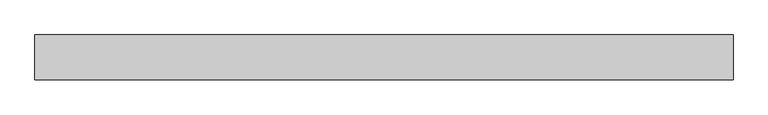
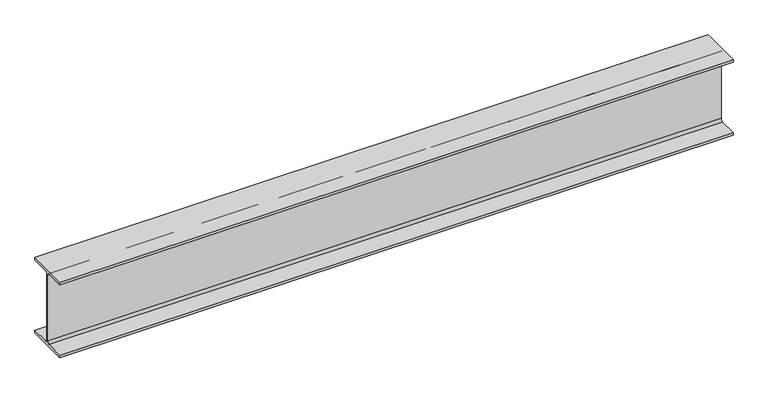
"""IFC4 building model written with IfcOpenShell, lengths in millimetres: beam geometry, Old_Steel Beam_H-KSD3502 : H_SB_ASB_H-350×175x7x11."""

import ifcopenshell
import ifcopenshell.guid

model = None  # the IFC model being written
_history = None  # IfcOwnerHistory: only IFC2X3 demands one
_inside = {}  # id of a spatial element -> (the spatial element, [elements in it])
_under = {}  # id of a project, library or spatial element -> (it, [spatial elements below it])
_declared = {}  # id of a project -> (the project, [libraries it declares])
_typed = {}  # id of a type object -> (the type object, [elements of that type])
_made_of = {}  # id of a material, layer set ... -> (it, [elements and type objects made of it])


def new_model(schema):
    """Start an empty IFC model of exactly this schema.

    Asked for "IFC4X3", IfcOpenShell would pick the latest addendum, in which some entities
    have other attributes; the version numbers below select the first issue.
    IFC2X3 requires an IfcOwnerHistory on every rooted entity: one is made here for all.
    """
    global model, _history
    if schema == "IFC4X3":
        model = ifcopenshell.file(schema_version=(4, 3, 0, 0))
    else:
        model = ifcopenshell.file(schema=schema)
    _inside.clear()
    _under.clear()
    _declared.clear()
    _typed.clear()
    _made_of.clear()
    _history = None
    if model.schema == "IFC2X3":
        org = make("IfcOrganization", Name="unknown")
        user = make(
            "IfcPersonAndOrganization",
            ThePerson=make("IfcPerson", FamilyName="unknown"),
            TheOrganization=org,
        )
        app = make(
            "IfcApplication",
            ApplicationDeveloper=org,
            Version="unknown",
            ApplicationFullName="unknown",
            ApplicationIdentifier="unknown",
        )
        _history = make(
            "IfcOwnerHistory",
            OwningUser=user,
            OwningApplication=app,
            ChangeAction="ADDED",
            CreationDate=0,
        )
    return model


def make(cls, **values):
    """One entity of the class cls with the attributes given. An attribute that is None is left unset."""
    return model.create_entity(
        cls, **{name: value for name, value in values.items() if value is not None}
    )


def rooted(cls, **values):
    """An entity with a GlobalId (a new one), such as an element, a storey or a relation."""
    return make(cls, GlobalId=ifcopenshell.guid.new(), OwnerHistory=_history, **values)


def si_unit(unit_type, name, prefix=None):
    """IfcSIUnit, for example si_unit("LENGTHUNIT", "METRE", prefix="MILLI")."""
    return make("IfcSIUnit", UnitType=unit_type, Prefix=prefix, Name=name)


def assignment(units):
    """IfcUnitAssignment: the units of a project."""
    return None if units is None else make("IfcUnitAssignment", Units=units)


def point(xyz):
    """IfcCartesianPoint."""
    return None if xyz is None else make("IfcCartesianPoint", Coordinates=xyz)


def direction(xyz):
    """IfcDirection."""
    return None if xyz is None else make("IfcDirection", DirectionRatios=xyz)


def frame(location, z_axis=None, x_axis=None):
    """IfcAxis2Placement3D, a coordinate frame: its origin and axes. An axis left out is left unset."""
    return make(
        "IfcAxis2Placement3D",
        Location=point(location),
        Axis=direction(z_axis),
        RefDirection=direction(x_axis),
    )


def frame_2d(location, x_axis=None):
    """IfcAxis2Placement2D, a coordinate frame in the plane: its origin and x axis."""
    return make(
        "IfcAxis2Placement2D", Location=point(location), RefDirection=direction(x_axis)
    )


def origin():
    """The frame at (0, 0, 0) with its axes left unset."""
    return frame((0.0, 0.0, 0.0))


def place(relative_to, where):
    """IfcLocalPlacement: puts the frame where relative to a parent placement (None: the world)."""
    return make(
        "IfcLocalPlacement", PlacementRelTo=relative_to, RelativePlacement=where
    )


def context(
    kind, dimensions, precision=None, world=None, true_north=None, identifier=None
):
    """IfcGeometricRepresentationContext, for example the 3D "Model" context."""
    return make(
        "IfcGeometricRepresentationContext",
        ContextIdentifier=identifier,
        ContextType=kind,
        CoordinateSpaceDimension=dimensions,
        Precision=precision,
        WorldCoordinateSystem=world,
        TrueNorth=true_north,
    )


def project(units=None, contexts=None):
    """IfcProject with its units and contexts."""
    return rooted(
        "IfcProject",
        Name="project",
        RepresentationContexts=contexts,
        UnitsInContext=assignment(units),
    )


def spatial(cls, under=None, at=None, **own):
    """A site, building, storey or space (cls), placed at a placement, below another one or the project."""
    s = rooted(cls, ObjectPlacement=at, **own)
    if under is not None:
        _under.setdefault(under.id(), (under, []))[1].append(s)
    return s


def polyline(points):
    """IfcPolyline through the points."""
    return make("IfcPolyline", Points=[point(p) for p in points])


def circle_curve(where, radius):
    """IfcCircle in the frame where."""
    return make("IfcCircle", Position=where, Radius=radius)


def trimmed(basis, trim1, trim2, sense, master):
    """IfcTrimmedCurve: the piece of a basis curve between two trims."""
    return make(
        "IfcTrimmedCurve",
        BasisCurve=basis,
        Trim1=trim1,
        Trim2=trim2,
        SenseAgreement=sense,
        MasterRepresentation=master,
    )


def segment(curve, same_sense, transition):
    """IfcCompositeCurveSegment."""
    return make(
        "IfcCompositeCurveSegment",
        Transition=transition,
        SameSense=same_sense,
        ParentCurve=curve,
    )


def composite_curve(segments, self_intersect=None):
    """IfcCompositeCurve: segments joined end to end."""
    return make("IfcCompositeCurve", Segments=segments, SelfIntersect=self_intersect)


def outline(outer, holes=None, kind="AREA"):
    """IfcArbitraryClosedProfileDef: a profile drawn as a closed curve; with holes, ...WithVoids."""
    if holes is None:
        return make("IfcArbitraryClosedProfileDef", ProfileType=kind, OuterCurve=outer)
    return make(
        "IfcArbitraryProfileDefWithVoids",
        ProfileType=kind,
        OuterCurve=outer,
        InnerCurves=holes,
    )


def extrude(swept, where, along, depth):
    """IfcExtrudedAreaSolid: the profile swept, set in the frame where, extruded along a direction by depth."""
    return make(
        "IfcExtrudedAreaSolid",
        SweptArea=swept,
        Position=where,
        ExtrudedDirection=direction(along),
        Depth=depth,
    )


def shape(context_of_items, identifier, shape_type, items):
    """IfcShapeRepresentation: the items that make up one representation, for example the "Body"."""
    return make(
        "IfcShapeRepresentation",
        ContextOfItems=context_of_items,
        RepresentationIdentifier=identifier,
        RepresentationType=shape_type,
        Items=items,
    )


def source(mapping_origin, context_of_items, identifier, shape_type, items):
    """IfcRepresentationMap: a shape defined once, which mapped items show again and again."""
    return make(
        "IfcRepresentationMap",
        MappingOrigin=mapping_origin,
        MappedRepresentation=shape(context_of_items, identifier, shape_type, items),
    )


def transform(
    local_origin,
    x_axis=None,
    y_axis=None,
    z_axis=None,
    scale=None,
    scale2=None,
    scale3=None,
    uniform=True,
):
    """IfcCartesianTransformationOperator3D, or its non-uniform kind. x_axis, y_axis, z_axis: its Axis1, 2, 3."""
    if uniform:
        return make(
            "IfcCartesianTransformationOperator3D",
            Axis1=direction(x_axis),
            Axis2=direction(y_axis),
            LocalOrigin=point(local_origin),
            Scale=scale,
            Axis3=direction(z_axis),
        )
    return make(
        "IfcCartesianTransformationOperator3DnonUniform",
        Axis1=direction(x_axis),
        Axis2=direction(y_axis),
        LocalOrigin=point(local_origin),
        Scale=scale,
        Axis3=direction(z_axis),
        Scale2=scale2,
        Scale3=scale3,
    )


def mapped(mapping_source, mapping_target):
    """IfcMappedItem: shows the shape of a source again, moved by a transform."""
    return make(
        "IfcMappedItem", MappingSource=mapping_source, MappingTarget=mapping_target
    )


def made_of(thing, what):
    """Note that an element or type object is made of a material, layer set ...; save() writes the relation."""
    if what is not None:
        _made_of.setdefault(what.id(), (what, []))[1].append(thing)
    return thing


def element(
    cls,
    number,
    at=None,
    inside=None,
    cuts=None,
    type_object=None,
    material=None,
    context=None,
    identifier="Body",
    shape_type=None,
    held_by="IfcProductDefinitionShape",
    body=None,
    shapes=None,
    **own,
):
    """One element of the class cls, such as IfcWall. Its Tag is "e" and its number.

    at: its placement. inside: the storey or other place that contains it. cuts: it is an
    opening in that element (IfcRelVoidsElement). A single representation is given by context,
    identifier, shape_type and body (its items); several are given by shapes. held_by: the class
    of the entity that holds the representations. save() writes the other relations.
    """
    e = rooted(cls, Tag="e%d" % number, ObjectPlacement=at, **own)
    if body is not None:
        shapes = [shape(context, identifier, shape_type, body)]
    if shapes is not None:
        e.Representation = make(held_by, Representations=shapes)
    if inside is not None:
        _inside.setdefault(inside.id(), (inside, []))[1].append(e)
    if cuts is not None:
        rooted(
            "IfcRelVoidsElement", RelatingBuildingElement=cuts, RelatedOpeningElement=e
        )
    if type_object is not None:
        _typed.setdefault(type_object.id(), (type_object, []))[1].append(e)
    return made_of(e, material)


def aggregate(whole, parts):
    """IfcRelAggregates: a whole, such as a stair, and the parts it consists of."""
    return rooted("IfcRelAggregates", RelatingObject=whole, RelatedObjects=parts)


def save(model, path):
    """Write the relations noted so far, then the file.

    IfcRelAggregates (storeys below a building ...), IfcRelContainedInSpatialStructure (elements
    in a storey), IfcRelDefinesByType, IfcRelAssociatesMaterial and IfcRelDeclares: one each for
    every whole, place, type object, material and project.
    """
    for whole, parts in _under.values():
        aggregate(whole, parts)
    for where, things in _inside.values():
        rooted(
            "IfcRelContainedInSpatialStructure",
            RelatedElements=things,
            RelatingStructure=where,
        )
    for kind, things in _typed.values():
        rooted("IfcRelDefinesByType", RelatedObjects=things, RelatingType=kind)
    for what, things in _made_of.values():
        rooted("IfcRelAssociatesMaterial", RelatedObjects=things, RelatingMaterial=what)
    for by, libraries in _declared.values():
        rooted("IfcRelDeclares", RelatingContext=by, RelatedDefinitions=libraries)
    model.write(path)


def beam_d6e73aa4(model_context):
    return source(origin(), model_context, "Body", "SweptSolid", [
        extrude(outline(composite_curve([segment(polyline([(82.5, -141.5), (82.5, -151.7), (-82.5, -151.7), (-82.5, -141.5), (-11.9, -141.5)]), True, "CONTINUOUS"), segment(trimmed(circle_curve(frame_2d((-11.9, -132.6)), 8.9), [point((-11.9, -141.5))], [point((-3.0, -132.6))], True, "CARTESIAN"), True, "CONTINUOUS"), segment(polyline([(-3.0, -132.6), (-3.0, 132.6)]), True, "CONTINUOUS"), segment(trimmed(circle_curve(frame_2d((-11.9, 132.6)), 8.9), [point((-3.0, 132.6))], [point((-11.9, 141.5))], True, "CARTESIAN"), True, "CONTINUOUS"), segment(polyline([(-11.9, 141.5), (-82.5, 141.5), (-82.5, 151.7), (82.5, 151.7), (82.5, 141.5), (11.9, 141.5)]), True, "CONTINUOUS"), segment(trimmed(circle_curve(frame_2d((11.9, 132.6)), 8.9), [point((11.9, 141.5))], [point((3.0, 132.6))], True, "CARTESIAN"), True, "CONTINUOUS"), segment(polyline([(3.0, 132.6), (3.0, -132.6)]), True, "CONTINUOUS"), segment(trimmed(circle_curve(frame_2d((11.9, -132.6)), 8.9), [point((3.0, -132.6))], [point((11.9, -141.5))], True, "CARTESIAN"), True, "CONTINUOUS"), segment(polyline([(11.9, -141.5), (82.5, -141.5)]), True, "CONTINUOUS")], self_intersect=False)), frame((-1265.9227894, 0.0, 0.0), z_axis=(1.0, 0.0, 0.0), x_axis=(0.0, 1.0, 0.0)), (0.0, 0.0, 1.0), 2561.6966945),
    ])


if __name__ == "__main__":
    model = new_model("IFC4")
    model_context = context("Model", 3, world=origin())
    ifc_project = project(units=[si_unit("LENGTHUNIT", "METRE", prefix="MILLI")], contexts=[model_context])
    site = spatial("IfcSite", under=ifc_project)
    building = spatial("IfcBuilding", under=site)
    placement = place(None, origin())
    beam_shape = beam_d6e73aa4(model_context)
    element("IfcBeam", 1, ObjectType="Old_Steel Beam_H-KSD3502 : H_SB_ASB_H-350×175x7x11", at=placement, inside=building, context=model_context, shape_type="MappedRepresentation", body=[
        mapped(beam_shape, transform((0.0, 0.0, 0.0), x_axis=(1.0, 0.0, 0.0), y_axis=(0.0, 1.0, 0.0), z_axis=(0.0, 0.0, 1.0))),
    ])
    save(model, "model.ifc")

# Revit data of these elements
# Type "Old_Steel Beam_H-KSD3502 : H_SB_ASB_H-350×175x7x11"
#   Width = 17.5 cm
#   Web Thickness = 0.7 cm
#   Web Fillet = 1.4 cm
#   Warping Constant = 282290.0 cm⁶
#   Torsional Moment of Inertia = 19.4042 cm⁴
#   Torsional Modulus = 1.0 cm³
#   Section Area = 63.14 cm²
#   Plastic Modulus weak axis = 174.0 cm³
#   Plastic Modulus strong axis = 868.0 cm³
#   Perimeter = 1.36 m²/m
#   Nominal Weight = 49.60 kgf/m
#   Moment of Inertia weak axis = 984.00 cm⁴
#   Moment of Inertia strong axis = 13600.00 cm⁴
#   Height = 35.0 cm
#   Flange Thickness = 1.1 cm
#   Elastic Modulus weak axis = 112.0 cm³
#   Elastic Modulus strong axis = 775.0 cm³
#   Centroid Vertical = 17.5 cm
#   Centroid Horizontal = 8.75 cm
#   Length [instance default] = 1.5240 m
#   Structural Material [instance default] = Steel, 45-345
#   Assembly Code = ""
# Element 1 (IfcBeam, "Old_Steel Beam_H-KSD3502 : H_SB_ASB_H-350×175x7x11")
#   Structural Material = none
# Materials
#   "Steel, 45-345": class "Metal", colour RGB 189 187 185, transparency 0, Description = "Steel 345 MPa", Cost = 0
